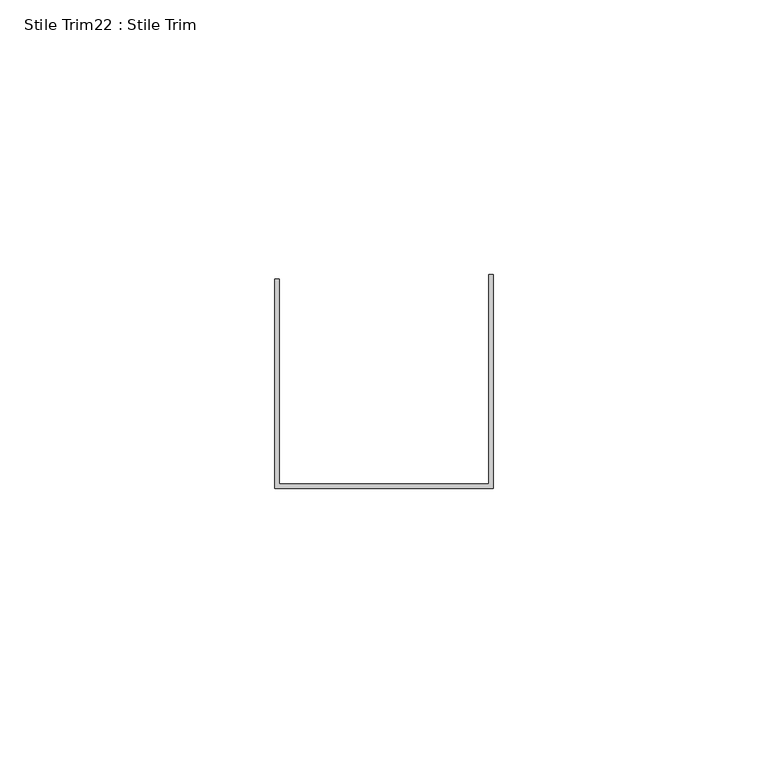
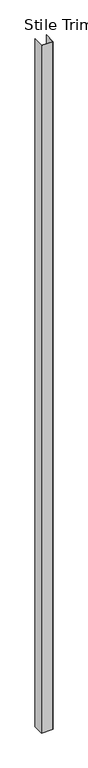
"""IFC4 building model written with IfcOpenShell, lengths in millimetres: proxy geometry, Stile Trim22 : Stile Trim."""

import ifcopenshell
import ifcopenshell.guid

model = None  # the IFC model being written
_history = None  # IfcOwnerHistory: only IFC2X3 demands one
_inside = {}  # id of a spatial element -> (the spatial element, [elements in it])
_under = {}  # id of a project, library or spatial element -> (it, [spatial elements below it])
_declared = {}  # id of a project -> (the project, [libraries it declares])
_typed = {}  # id of a type object -> (the type object, [elements of that type])
_made_of = {}  # id of a material, layer set ... -> (it, [elements and type objects made of it])


def new_model(schema):
    """Start an empty IFC model of exactly this schema.

    Asked for "IFC4X3", IfcOpenShell would pick the latest addendum, in which some entities
    have other attributes; the version numbers below select the first issue.
    IFC2X3 requires an IfcOwnerHistory on every rooted entity: one is made here for all.
    """
    global model, _history
    if schema == "IFC4X3":
        model = ifcopenshell.file(schema_version=(4, 3, 0, 0))
    else:
        model = ifcopenshell.file(schema=schema)
    _inside.clear()
    _under.clear()
    _declared.clear()
    _typed.clear()
    _made_of.clear()
    _history = None
    if model.schema == "IFC2X3":
        org = make("IfcOrganization", Name="unknown")
        user = make(
            "IfcPersonAndOrganization",
            ThePerson=make("IfcPerson", FamilyName="unknown"),
            TheOrganization=org,
        )
        app = make(
            "IfcApplication",
            ApplicationDeveloper=org,
            Version="unknown",
            ApplicationFullName="unknown",
            ApplicationIdentifier="unknown",
        )
        _history = make(
            "IfcOwnerHistory",
            OwningUser=user,
            OwningApplication=app,
            ChangeAction="ADDED",
            CreationDate=0,
        )
    return model


def make(cls, **values):
    """One entity of the class cls with the attributes given. An attribute that is None is left unset."""
    return model.create_entity(
        cls, **{name: value for name, value in values.items() if value is not None}
    )


def rooted(cls, **values):
    """An entity with a GlobalId (a new one), such as an element, a storey or a relation."""
    return make(cls, GlobalId=ifcopenshell.guid.new(), OwnerHistory=_history, **values)


def si_unit(unit_type, name, prefix=None):
    """IfcSIUnit, for example si_unit("LENGTHUNIT", "METRE", prefix="MILLI")."""
    return make("IfcSIUnit", UnitType=unit_type, Prefix=prefix, Name=name)


def assignment(units):
    """IfcUnitAssignment: the units of a project."""
    return None if units is None else make("IfcUnitAssignment", Units=units)


def point(xyz):
    """IfcCartesianPoint."""
    return None if xyz is None else make("IfcCartesianPoint", Coordinates=xyz)


def direction(xyz):
    """IfcDirection."""
    return None if xyz is None else make("IfcDirection", DirectionRatios=xyz)


def frame(location, z_axis=None, x_axis=None):
    """IfcAxis2Placement3D, a coordinate frame: its origin and axes. An axis left out is left unset."""
    return make(
        "IfcAxis2Placement3D",
        Location=point(location),
        Axis=direction(z_axis),
        RefDirection=direction(x_axis),
    )


def origin():
    """The frame at (0, 0, 0) with its axes left unset."""
    return frame((0.0, 0.0, 0.0))


def origin_with_axes():
    """The frame at (0, 0, 0) with the z axis (0, 0, 1) and the x axis (1, 0, 0) written out."""
    return frame((0.0, 0.0, 0.0), z_axis=(0.0, 0.0, 1.0), x_axis=(1.0, 0.0, 0.0))


def place(relative_to, where):
    """IfcLocalPlacement: puts the frame where relative to a parent placement (None: the world)."""
    return make(
        "IfcLocalPlacement", PlacementRelTo=relative_to, RelativePlacement=where
    )


def context(
    kind, dimensions, precision=None, world=None, true_north=None, identifier=None
):
    """IfcGeometricRepresentationContext, for example the 3D "Model" context."""
    return make(
        "IfcGeometricRepresentationContext",
        ContextIdentifier=identifier,
        ContextType=kind,
        CoordinateSpaceDimension=dimensions,
        Precision=precision,
        WorldCoordinateSystem=world,
        TrueNorth=true_north,
    )


def project(units=None, contexts=None):
    """IfcProject with its units and contexts."""
    return rooted(
        "IfcProject",
        Name="project",
        RepresentationContexts=contexts,
        UnitsInContext=assignment(units),
    )


def spatial(cls, under=None, at=None, **own):
    """A site, building, storey or space (cls), placed at a placement, below another one or the project."""
    s = rooted(cls, ObjectPlacement=at, **own)
    if under is not None:
        _under.setdefault(under.id(), (under, []))[1].append(s)
    return s


def polyline(points):
    """IfcPolyline through the points."""
    return make("IfcPolyline", Points=[point(p) for p in points])


def outline(outer, holes=None, kind="AREA"):
    """IfcArbitraryClosedProfileDef: a profile drawn as a closed curve; with holes, ...WithVoids."""
    if holes is None:
        return make("IfcArbitraryClosedProfileDef", ProfileType=kind, OuterCurve=outer)
    return make(
        "IfcArbitraryProfileDefWithVoids",
        ProfileType=kind,
        OuterCurve=outer,
        InnerCurves=holes,
    )


def extrude(swept, where, along, depth):
    """IfcExtrudedAreaSolid: the profile swept, set in the frame where, extruded along a direction by depth."""
    return make(
        "IfcExtrudedAreaSolid",
        SweptArea=swept,
        Position=where,
        ExtrudedDirection=direction(along),
        Depth=depth,
    )


def shape(context_of_items, identifier, shape_type, items):
    """IfcShapeRepresentation: the items that make up one representation, for example the "Body"."""
    return make(
        "IfcShapeRepresentation",
        ContextOfItems=context_of_items,
        RepresentationIdentifier=identifier,
        RepresentationType=shape_type,
        Items=items,
    )


def source(mapping_origin, context_of_items, identifier, shape_type, items):
    """IfcRepresentationMap: a shape defined once, which mapped items show again and again."""
    return make(
        "IfcRepresentationMap",
        MappingOrigin=mapping_origin,
        MappedRepresentation=shape(context_of_items, identifier, shape_type, items),
    )


def transform(
    local_origin,
    x_axis=None,
    y_axis=None,
    z_axis=None,
    scale=None,
    scale2=None,
    scale3=None,
    uniform=True,
):
    """IfcCartesianTransformationOperator3D, or its non-uniform kind. x_axis, y_axis, z_axis: its Axis1, 2, 3."""
    if uniform:
        return make(
            "IfcCartesianTransformationOperator3D",
            Axis1=direction(x_axis),
            Axis2=direction(y_axis),
            LocalOrigin=point(local_origin),
            Scale=scale,
            Axis3=direction(z_axis),
        )
    return make(
        "IfcCartesianTransformationOperator3DnonUniform",
        Axis1=direction(x_axis),
        Axis2=direction(y_axis),
        LocalOrigin=point(local_origin),
        Scale=scale,
        Axis3=direction(z_axis),
        Scale2=scale2,
        Scale3=scale3,
    )


def mapped(mapping_source, mapping_target):
    """IfcMappedItem: shows the shape of a source again, moved by a transform."""
    return make(
        "IfcMappedItem", MappingSource=mapping_source, MappingTarget=mapping_target
    )


def made_of(thing, what):
    """Note that an element or type object is made of a material, layer set ...; save() writes the relation."""
    if what is not None:
        _made_of.setdefault(what.id(), (what, []))[1].append(thing)
    return thing


def element(
    cls,
    number,
    at=None,
    inside=None,
    cuts=None,
    type_object=None,
    material=None,
    context=None,
    identifier="Body",
    shape_type=None,
    held_by="IfcProductDefinitionShape",
    body=None,
    shapes=None,
    **own,
):
    """One element of the class cls, such as IfcWall. Its Tag is "e" and its number.

    at: its placement. inside: the storey or other place that contains it. cuts: it is an
    opening in that element (IfcRelVoidsElement). A single representation is given by context,
    identifier, shape_type and body (its items); several are given by shapes. held_by: the class
    of the entity that holds the representations. save() writes the other relations.
    """
    e = rooted(cls, Tag="e%d" % number, ObjectPlacement=at, **own)
    if body is not None:
        shapes = [shape(context, identifier, shape_type, body)]
    if shapes is not None:
        e.Representation = make(held_by, Representations=shapes)
    if inside is not None:
        _inside.setdefault(inside.id(), (inside, []))[1].append(e)
    if cuts is not None:
        rooted(
            "IfcRelVoidsElement", RelatingBuildingElement=cuts, RelatedOpeningElement=e
        )
    if type_object is not None:
        _typed.setdefault(type_object.id(), (type_object, []))[1].append(e)
    return made_of(e, material)


def aggregate(whole, parts):
    """IfcRelAggregates: a whole, such as a stair, and the parts it consists of."""
    return rooted("IfcRelAggregates", RelatingObject=whole, RelatedObjects=parts)


def save(model, path):
    """Write the relations noted so far, then the file.

    IfcRelAggregates (storeys below a building ...), IfcRelContainedInSpatialStructure (elements
    in a storey), IfcRelDefinesByType, IfcRelAssociatesMaterial and IfcRelDeclares: one each for
    every whole, place, type object, material and project.
    """
    for whole, parts in _under.values():
        aggregate(whole, parts)
    for where, things in _inside.values():
        rooted(
            "IfcRelContainedInSpatialStructure",
            RelatedElements=things,
            RelatingStructure=where,
        )
    for kind, things in _typed.values():
        rooted("IfcRelDefinesByType", RelatedObjects=things, RelatingType=kind)
    for what, things in _made_of.values():
        rooted("IfcRelAssociatesMaterial", RelatedObjects=things, RelatingMaterial=what)
    for by, libraries in _declared.values():
        rooted("IfcRelDeclares", RelatingContext=by, RelatedDefinitions=libraries)
    model.write(path)


def stile_trim22_stile_trim_a5a4c22f(model_context):
    return source(origin(), model_context, "Body", "SweptSolid", [
        extrude(outline(polyline([(590392.4558739, -536420.7663841), (590352.7810739, -536420.7663841), (590352.7810739, -536382.6663841), (590353.5684739, -536382.6663841), (590353.5684739, -536419.9789841), (590391.6684739, -536419.9789841), (590391.6684739, -536381.8789841), (590392.4558739, -536381.8789841), (590392.4558739, -536420.7663841)])), origin_with_axes(), (0.0, 0.0, 1.0), 2438.4),
    ])


if __name__ == "__main__":
    model = new_model("IFC4")
    model_context = context("Model", 3, world=origin())
    ifc_project = project(units=[si_unit("LENGTHUNIT", "METRE", prefix="MILLI")], contexts=[model_context])
    site = spatial("IfcSite", under=ifc_project)
    building = spatial("IfcBuilding", under=site)
    placement = place(None, origin())
    stile_trim22_stile_trim_shape = stile_trim22_stile_trim_a5a4c22f(model_context)
    element("IfcBuildingElementProxy", 1, Name="Stile Trim22 : Stile Trim", ObjectType="Stile Trim22 : Stile Trim", at=placement, inside=building, context=model_context, shape_type="MappedRepresentation", body=[
        mapped(stile_trim22_stile_trim_shape, transform((0.0, 0.0, 0.0), x_axis=(1.0, 0.0, 0.0), y_axis=(0.0, 1.0, 0.0), z_axis=(0.0, 0.0, 1.0))),
    ])
    save(model, "model.ifc")

# Revit data of these elements
# Element 1 (IfcBuildingElementProxy, "Stile Trim22 : Stile Trim")
#   Materials on its faces: "EDGE TRIM BY MTL PANEL MFR."
# Materials
#   "EDGE TRIM BY MTL PANEL MFR.": class "Generic", colour RGB 239 242 240, transparency 0, Cost = 0
